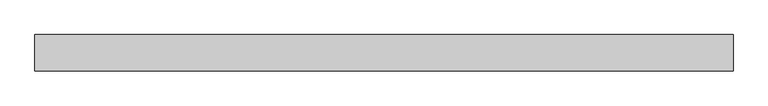
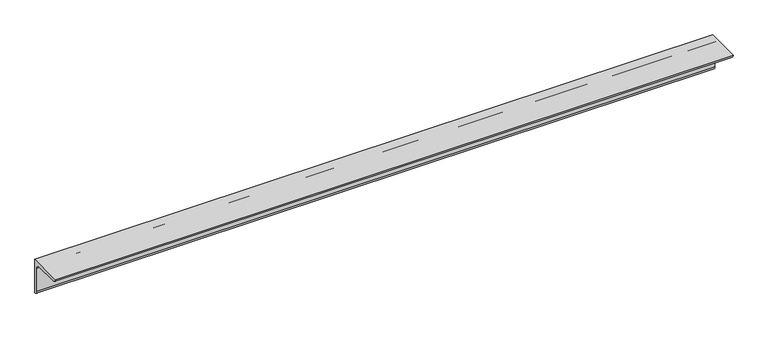
"""IFC4 building model written with IfcOpenShell, lengths in millimetres: member geometry, 0912_Steel Framing_L-KSD3502 : H_SB_AR_S04_L-100x100x10_KBR2."""

from ifc_helpers import new_model, si_unit, point, frame, frame_2d, origin, place, context, project, spatial, polyline, circle_curve, trimmed, segment, composite_curve, outline, extrude, source, transform, mapped, element, save


def member_98705e42(model_context):
    return source(origin(), model_context, "Body", "SweptSolid", [
        extrude(outline(composite_curve([segment(polyline([(28.2, 28.2), (28.2, -71.8)]), True, "CONTINUOUS"), segment(trimmed(circle_curve(frame_2d((28.2, -61.8)), 10.0), [point((28.2, -71.8))], [point((18.2, -61.8))], False, "CARTESIAN"), True, "CONTINUOUS"), segment(polyline([(18.2, -61.8), (18.2, 8.2)]), True, "CONTINUOUS"), segment(trimmed(circle_curve(frame_2d((8.2, 8.2)), 10.0), [point((18.2, 8.2))], [point((8.2, 18.2))], True, "CARTESIAN"), True, "CONTINUOUS"), segment(polyline([(8.2, 18.2), (-61.8, 18.2)]), True, "CONTINUOUS"), segment(trimmed(circle_curve(frame_2d((-61.8, 28.2)), 10.0), [point((-61.8, 18.2))], [point((-71.8, 28.2))], False, "CARTESIAN"), True, "CONTINUOUS"), segment(polyline([(-71.8, 28.2), (28.2, 28.2)]), True, "CONTINUOUS")], self_intersect=False)), frame((-925.8352801, 0.0, 0.0), z_axis=(1.0, 0.0, 0.0), x_axis=(0.0, 1.0, 0.0)), (0.0, 0.0, 1.0), 1920.9670248),
    ])


if __name__ == "__main__":
    model = new_model("IFC4")
    model_context = context("Model", 3, world=origin())
    ifc_project = project(units=[si_unit("LENGTHUNIT", "METRE", prefix="MILLI")], contexts=[model_context])
    site = spatial("IfcSite", under=ifc_project)
    building = spatial("IfcBuilding", under=site)
    placement = place(None, origin())
    member_shape = member_98705e42(model_context)
    element("IfcMember", 1, ObjectType="0912_Steel Framing_L-KSD3502 : H_SB_AR_S04_L-100x100x10_KBR2", at=placement, inside=building, context=model_context, shape_type="MappedRepresentation", body=[
        mapped(member_shape, transform((0.0, 0.0, 0.0), x_axis=(1.0, 0.0, 0.0), y_axis=(0.0, 1.0, 0.0), z_axis=(0.0, 0.0, 1.0))),
    ])
    save(model, "model.ifc")

# Revit data of these elements
# Type "0912_Steel Framing_L-KSD3502 : H_SB_AR_S04_L-100x100x10_KBR2"
#   k = 25 mm
#   Perimeter = 0.40 m²/m
#   Nominal Weight = 14.90 kgf/m
#   Length [instance default] = 1000 mm
#   b = 100 mm
#   d = 100 mm
#   t = 10 mm
#   x = 28.2 mm
#   y = 28.2 mm
#   A = 1900.00 m²
#   Structural Material [instance default] = Steel, 45-345
# Element 1 (IfcMember, "0912_Steel Framing_L-KSD3502 : H_SB_AR_S04_L-100x100x10_KBR2")
#   Materials on its faces: "Steel, 45-345"
# Materials
#   "Steel, 45-345": class "Metal", colour RGB 189 187 185, transparency 0, Description = "Steel 345 MPa", Cost = 0
